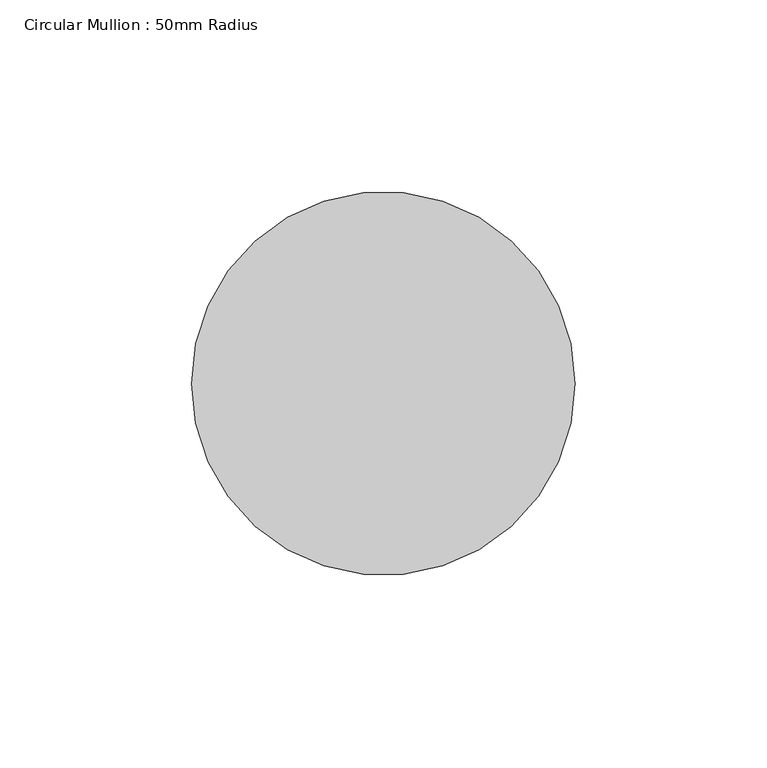
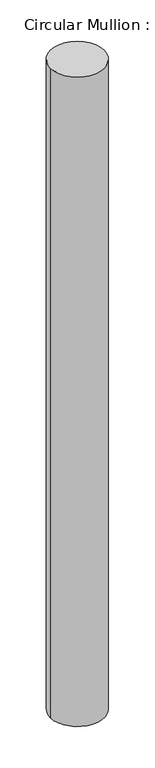
"""IFC4 building model written with IfcOpenShell, lengths in millimetres: member geometry, Circular Mullion : 50mm Radius."""

from ifc_helpers import new_model, si_unit, point, frame, origin, origin_2d, place, context, project, spatial, circle_curve, trimmed, segment, composite_curve, outline, extrude, source, transform, mapped, element, save


def circular_mullion_50mm_radius_3157869f(model_context):
    return source(origin(), model_context, "Body", "SweptSolid", [
        extrude(outline(composite_curve([segment(trimmed(circle_curve(origin_2d(), 50.0), [point((50.0, 0.0))], [point((-50.0, 0.0))], False, "CARTESIAN"), True, "CONTINUOUS"), segment(trimmed(circle_curve(origin_2d(), 50.0), [point((-50.0, 0.0))], [point((50.0, 0.0))], False, "CARTESIAN"), True, "CONTINUOUS")], self_intersect=False)), frame((0.0, 0.0, -1276.3088296), z_axis=(0.0, 0.0, 1.0), x_axis=(1.0, 0.0, 0.0)), (0.0, 0.0, 1.0), 1276.3088296),
    ])


if __name__ == "__main__":
    model = new_model("IFC4")
    model_context = context("Model", 3, world=origin())
    ifc_project = project(units=[si_unit("LENGTHUNIT", "METRE", prefix="MILLI")], contexts=[model_context])
    site = spatial("IfcSite", under=ifc_project)
    building = spatial("IfcBuilding", under=site)
    placement = place(None, origin())
    circular_mullion_50mm_radius_shape = circular_mullion_50mm_radius_3157869f(model_context)
    element("IfcMember", 1, ObjectType="Circular Mullion : 50mm Radius", at=placement, inside=building, context=model_context, shape_type="MappedRepresentation", body=[
        mapped(circular_mullion_50mm_radius_shape, transform((0.0, 0.0, 0.0), x_axis=(1.0, 0.0, 0.0), y_axis=(0.0, 1.0, 0.0), z_axis=(0.0, 0.0, 1.0))),
    ])
    save(model, "model.ifc")

# Revit data of these elements
# Type "Circular Mullion : 50mm Radius"
#   built-in parameter 1007350 = 0.164042 (stored number, unit not read)
# Element 1 (IfcMember, "Circular Mullion : 50mm Radius")
#   Materials on its faces: "Aluminium"
# Materials
#   "Aluminium": class "Metal", colour RGB 247 247 247, transparency 0, Description = "Aluminium 6061", Cost = 0
